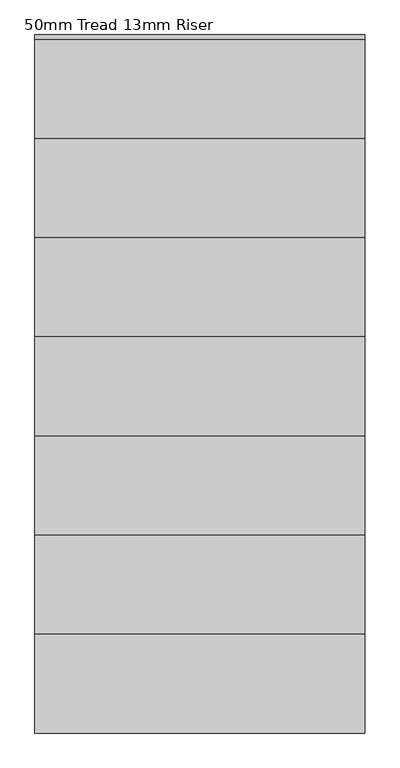
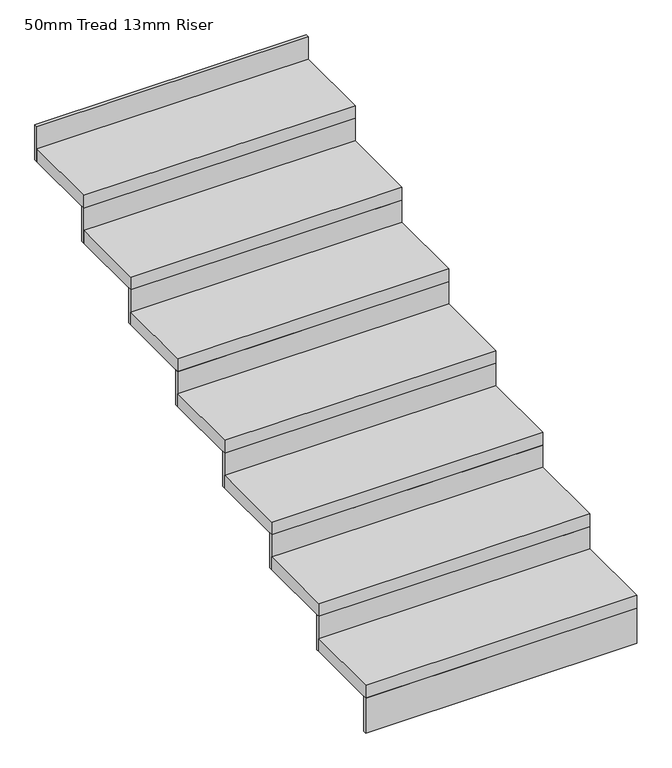
"""IFC4 building model written with IfcOpenShell, lengths in millimetres: stair flight geometry, 50mm Tread 13mm Riser."""

from ifc_helpers import new_model, si_unit, frame, origin, place, context, project, spatial, polyline, outline, extrude, source, transform, mapped, element, save


def stair_flight_50mm_tread_13mm_riser_a664a014(model_context):
    return source(origin(), model_context, "Body", "SweptSolid", [
        extrude(outline(polyline([(22549.836337, -1888.024372), (22549.836337, -1900.524372), (21549.836337, -1900.524372), (21549.836337, -1888.024372), (22549.836337, -1888.024372)])), frame((0.0, 0.0, 1859.0909091), z_axis=(0.0, 0.0, 1.0), x_axis=(1.0, 0.0, 0.0)), (0.0, 0.0, 1.0), 136.3636364),
        extrude(outline(polyline([(21549.836337, -1600.524372), (22549.836337, -1600.524372), (22549.836337, -1900.524372), (21549.836337, -1900.524372), (21549.836337, -1600.524372)])), frame((0.0, 0.0, 1995.4545455), z_axis=(0.0, 0.0, 1.0), x_axis=(1.0, 0.0, 0.0)), (0.0, 0.0, 1.0), 50.0),
        extrude(outline(polyline([(22549.836337, -1588.024372), (22549.836337, -1600.524372), (21549.836337, -1600.524372), (21549.836337, -1588.024372), (22549.836337, -1588.024372)])), frame((0.0, 0.0, 1995.4545455), z_axis=(0.0, 0.0, 1.0), x_axis=(1.0, 0.0, 0.0)), (0.0, 0.0, 1.0), 136.3636364),
        extrude(outline(polyline([(21549.836337, -1300.524372), (22549.836337, -1300.524372), (22549.836337, -1600.524372), (21549.836337, -1600.524372), (21549.836337, -1300.524372)])), frame((0.0, 0.0, 2131.8181818), z_axis=(0.0, 0.0, 1.0), x_axis=(1.0, 0.0, 0.0)), (0.0, 0.0, 1.0), 50.0),
        extrude(outline(polyline([(22549.836337, -1288.024372), (22549.836337, -1300.524372), (21549.836337, -1300.524372), (21549.836337, -1288.024372), (22549.836337, -1288.024372)])), frame((0.0, 0.0, 2131.8181818), z_axis=(0.0, 0.0, 1.0), x_axis=(1.0, 0.0, 0.0)), (0.0, 0.0, 1.0), 136.3636364),
        extrude(outline(polyline([(21549.836337, -1000.524372), (22549.836337, -1000.524372), (22549.836337, -1300.524372), (21549.836337, -1300.524372), (21549.836337, -1000.524372)])), frame((0.0, 0.0, 2268.1818182), z_axis=(0.0, 0.0, 1.0), x_axis=(1.0, 0.0, 0.0)), (0.0, 0.0, 1.0), 50.0),
        extrude(outline(polyline([(22549.836337, -988.024372), (22549.836337, -1000.524372), (21549.836337, -1000.524372), (21549.836337, -988.024372), (22549.836337, -988.024372)])), frame((0.0, 0.0, 2268.1818182), z_axis=(0.0, 0.0, 1.0), x_axis=(1.0, 0.0, 0.0)), (0.0, 0.0, 1.0), 136.3636364),
        extrude(outline(polyline([(21549.836337, -700.524372), (22549.836337, -700.524372), (22549.836337, -1000.524372), (21549.836337, -1000.524372), (21549.836337, -700.524372)])), frame((0.0, 0.0, 2404.5454545), z_axis=(0.0, 0.0, 1.0), x_axis=(1.0, 0.0, 0.0)), (0.0, 0.0, 1.0), 50.0),
        extrude(outline(polyline([(22549.836337, -688.024372), (22549.836337, -700.524372), (21549.836337, -700.524372), (21549.836337, -688.024372), (22549.836337, -688.024372)])), frame((0.0, 0.0, 2404.5454545), z_axis=(0.0, 0.0, 1.0), x_axis=(1.0, 0.0, 0.0)), (0.0, 0.0, 1.0), 136.3636364),
        extrude(outline(polyline([(21549.836337, -400.524372), (22549.836337, -400.524372), (22549.836337, -700.524372), (21549.836337, -700.524372), (21549.836337, -400.524372)])), frame((0.0, 0.0, 2540.9090909), z_axis=(0.0, 0.0, 1.0), x_axis=(1.0, 0.0, 0.0)), (0.0, 0.0, 1.0), 50.0),
        extrude(outline(polyline([(22549.836337, -388.024372), (22549.836337, -400.524372), (21549.836337, -400.524372), (21549.836337, -388.024372), (22549.836337, -388.024372)])), frame((0.0, 0.0, 2540.9090909), z_axis=(0.0, 0.0, 1.0), x_axis=(1.0, 0.0, 0.0)), (0.0, 0.0, 1.0), 136.3636364),
        extrude(outline(polyline([(21549.836337, -100.524372), (22549.836337, -100.524372), (22549.836337, -400.524372), (21549.836337, -400.524372), (21549.836337, -100.524372)])), frame((0.0, 0.0, 2677.2727273), z_axis=(0.0, 0.0, 1.0), x_axis=(1.0, 0.0, 0.0)), (0.0, 0.0, 1.0), 50.0),
        extrude(outline(polyline([(22549.836337, -88.024372), (22549.836337, -100.524372), (21549.836337, -100.524372), (21549.836337, -88.024372), (22549.836337, -88.024372)])), frame((0.0, 0.0, 2677.2727273), z_axis=(0.0, 0.0, 1.0), x_axis=(1.0, 0.0, 0.0)), (0.0, 0.0, 1.0), 136.3636364),
        extrude(outline(polyline([(21549.836337, 199.475628), (22549.836337, 199.475628), (22549.836337, -100.524372), (21549.836337, -100.524372), (21549.836337, 199.475628)])), frame((0.0, 0.0, 2813.6363636), z_axis=(0.0, 0.0, 1.0), x_axis=(1.0, 0.0, 0.0)), (0.0, 0.0, 1.0), 50.0),
        extrude(outline(polyline([(22549.836337, 211.975628), (22549.836337, 199.475628), (21549.836337, 199.475628), (21549.836337, 211.975628), (22549.836337, 211.975628)])), frame((0.0, 0.0, 2813.6363636), z_axis=(0.0, 0.0, 1.0), x_axis=(1.0, 0.0, 0.0)), (0.0, 0.0, 1.0), 136.3636364),
    ])


if __name__ == "__main__":
    model = new_model("IFC4")
    model_context = context("Model", 3, world=origin())
    ifc_project = project(units=[si_unit("LENGTHUNIT", "METRE", prefix="MILLI")], contexts=[model_context])
    site = spatial("IfcSite", under=ifc_project)
    building = spatial("IfcBuilding", under=site)
    placement = place(None, origin())
    stair_flight_50mm_tread_13mm_riser_shape = stair_flight_50mm_tread_13mm_riser_a664a014(model_context)
    element("IfcStairFlight", 1, ObjectType="50mm Tread 13mm Riser", at=placement, inside=building, context=model_context, shape_type="MappedRepresentation", body=[
        mapped(stair_flight_50mm_tread_13mm_riser_shape, transform((0.0, 0.0, 0.0), x_axis=(1.0, 0.0, 0.0), y_axis=(0.0, 1.0, 0.0), z_axis=(0.0, 0.0, 1.0))),
    ])
    save(model, "model.ifc")
